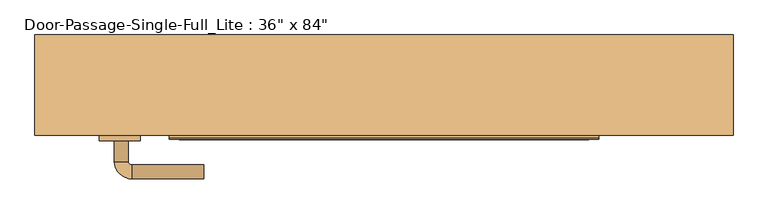
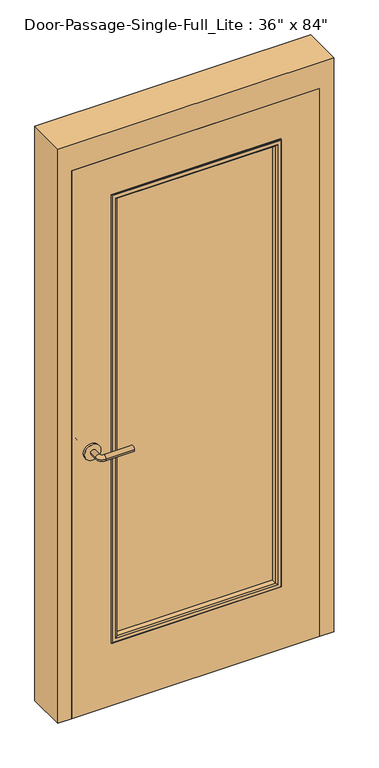
"""IFC4 building model written with IfcOpenShell, lengths in millimetres: door geometry."""

import ifcopenshell
import ifcopenshell.guid

model = None  # the IFC model being written
_history = None  # IfcOwnerHistory: only IFC2X3 demands one
_inside = {}  # id of a spatial element -> (the spatial element, [elements in it])
_under = {}  # id of a project, library or spatial element -> (it, [spatial elements below it])
_declared = {}  # id of a project -> (the project, [libraries it declares])
_typed = {}  # id of a type object -> (the type object, [elements of that type])
_made_of = {}  # id of a material, layer set ... -> (it, [elements and type objects made of it])


def new_model(schema):
    """Start an empty IFC model of exactly this schema.

    Asked for "IFC4X3", IfcOpenShell would pick the latest addendum, in which some entities
    have other attributes; the version numbers below select the first issue.
    IFC2X3 requires an IfcOwnerHistory on every rooted entity: one is made here for all.
    """
    global model, _history
    if schema == "IFC4X3":
        model = ifcopenshell.file(schema_version=(4, 3, 0, 0))
    else:
        model = ifcopenshell.file(schema=schema)
    _inside.clear()
    _under.clear()
    _declared.clear()
    _typed.clear()
    _made_of.clear()
    _history = None
    if model.schema == "IFC2X3":
        org = make("IfcOrganization", Name="unknown")
        user = make(
            "IfcPersonAndOrganization",
            ThePerson=make("IfcPerson", FamilyName="unknown"),
            TheOrganization=org,
        )
        app = make(
            "IfcApplication",
            ApplicationDeveloper=org,
            Version="unknown",
            ApplicationFullName="unknown",
            ApplicationIdentifier="unknown",
        )
        _history = make(
            "IfcOwnerHistory",
            OwningUser=user,
            OwningApplication=app,
            ChangeAction="ADDED",
            CreationDate=0,
        )
    return model


def make(cls, **values):
    """One entity of the class cls with the attributes given. An attribute that is None is left unset."""
    return model.create_entity(
        cls, **{name: value for name, value in values.items() if value is not None}
    )


def rooted(cls, **values):
    """An entity with a GlobalId (a new one), such as an element, a storey or a relation."""
    return make(cls, GlobalId=ifcopenshell.guid.new(), OwnerHistory=_history, **values)


def si_unit(unit_type, name, prefix=None):
    """IfcSIUnit, for example si_unit("LENGTHUNIT", "METRE", prefix="MILLI")."""
    return make("IfcSIUnit", UnitType=unit_type, Prefix=prefix, Name=name)


def assignment(units):
    """IfcUnitAssignment: the units of a project."""
    return None if units is None else make("IfcUnitAssignment", Units=units)


def point(xyz):
    """IfcCartesianPoint."""
    return None if xyz is None else make("IfcCartesianPoint", Coordinates=xyz)


def direction(xyz):
    """IfcDirection."""
    return None if xyz is None else make("IfcDirection", DirectionRatios=xyz)


def frame(location, z_axis=None, x_axis=None):
    """IfcAxis2Placement3D, a coordinate frame: its origin and axes. An axis left out is left unset."""
    return make(
        "IfcAxis2Placement3D",
        Location=point(location),
        Axis=direction(z_axis),
        RefDirection=direction(x_axis),
    )


def frame_2d(location, x_axis=None):
    """IfcAxis2Placement2D, a coordinate frame in the plane: its origin and x axis."""
    return make(
        "IfcAxis2Placement2D", Location=point(location), RefDirection=direction(x_axis)
    )


def origin():
    """The frame at (0, 0, 0) with its axes left unset."""
    return frame((0.0, 0.0, 0.0))


def place(relative_to, where):
    """IfcLocalPlacement: puts the frame where relative to a parent placement (None: the world)."""
    return make(
        "IfcLocalPlacement", PlacementRelTo=relative_to, RelativePlacement=where
    )


def context(
    kind, dimensions, precision=None, world=None, true_north=None, identifier=None
):
    """IfcGeometricRepresentationContext, for example the 3D "Model" context."""
    return make(
        "IfcGeometricRepresentationContext",
        ContextIdentifier=identifier,
        ContextType=kind,
        CoordinateSpaceDimension=dimensions,
        Precision=precision,
        WorldCoordinateSystem=world,
        TrueNorth=true_north,
    )


def project(units=None, contexts=None):
    """IfcProject with its units and contexts."""
    return rooted(
        "IfcProject",
        Name="project",
        RepresentationContexts=contexts,
        UnitsInContext=assignment(units),
    )


def spatial(cls, under=None, at=None, **own):
    """A site, building, storey or space (cls), placed at a placement, below another one or the project."""
    s = rooted(cls, ObjectPlacement=at, **own)
    if under is not None:
        _under.setdefault(under.id(), (under, []))[1].append(s)
    return s


def polyline(points):
    """IfcPolyline through the points."""
    return make("IfcPolyline", Points=[point(p) for p in points])


def circle_curve(where, radius):
    """IfcCircle in the frame where."""
    return make("IfcCircle", Position=where, Radius=radius)


def ellipse_curve(where, semi_axis1, semi_axis2):
    """IfcEllipse in the frame where."""
    return make(
        "IfcEllipse", Position=where, SemiAxis1=semi_axis1, SemiAxis2=semi_axis2
    )


def trimmed(basis, trim1, trim2, sense, master):
    """IfcTrimmedCurve: the piece of a basis curve between two trims."""
    return make(
        "IfcTrimmedCurve",
        BasisCurve=basis,
        Trim1=trim1,
        Trim2=trim2,
        SenseAgreement=sense,
        MasterRepresentation=master,
    )


def segment(curve, same_sense, transition):
    """IfcCompositeCurveSegment."""
    return make(
        "IfcCompositeCurveSegment",
        Transition=transition,
        SameSense=same_sense,
        ParentCurve=curve,
    )


def composite_curve(segments, self_intersect=None):
    """IfcCompositeCurve: segments joined end to end."""
    return make("IfcCompositeCurve", Segments=segments, SelfIntersect=self_intersect)


def outline(outer, holes=None, kind="AREA"):
    """IfcArbitraryClosedProfileDef: a profile drawn as a closed curve; with holes, ...WithVoids."""
    if holes is None:
        return make("IfcArbitraryClosedProfileDef", ProfileType=kind, OuterCurve=outer)
    return make(
        "IfcArbitraryProfileDefWithVoids",
        ProfileType=kind,
        OuterCurve=outer,
        InnerCurves=holes,
    )


def extrude(swept, where, along, depth):
    """IfcExtrudedAreaSolid: the profile swept, set in the frame where, extruded along a direction by depth."""
    return make(
        "IfcExtrudedAreaSolid",
        SweptArea=swept,
        Position=where,
        ExtrudedDirection=direction(along),
        Depth=depth,
    )


def faces_of(points, faces, orient=None, outer=None):
    """IfcFace entities. A face is a list of loops; a loop is a list of indices into points, from 0.

    orient and outer hold one flag for each loop. By default every Orientation is true, the
    first loop of a face is its IfcFaceOuterBound and the others are IfcFaceBound.
    """
    made = []
    for i, loops in enumerate(faces):
        bounds = []
        for j, loop in enumerate(loops):
            is_outer = j == 0 if outer is None else outer[i][j]
            bounds.append(
                make(
                    "IfcFaceOuterBound" if is_outer else "IfcFaceBound",
                    Bound=make("IfcPolyLoop", Polygon=[points[k] for k in loop]),
                    Orientation=True if orient is None else orient[i][j],
                )
            )
        made.append(make("IfcFace", Bounds=bounds))
    return made


def faceted_brep(points, faces, orient=None, outer=None, voids=None):
    """IfcFacetedBrep: a solid bounded by flat faces; with voids (closed shells), ...WithVoids."""
    shared = [point(p) for p in points]
    hull = make("IfcClosedShell", CfsFaces=faces_of(shared, faces, orient, outer))
    if voids is None:
        return make("IfcFacetedBrep", Outer=hull)
    return make(
        "IfcFacetedBrepWithVoids",
        Outer=hull,
        Voids=[
            make(cls, CfsFaces=faces_of(shared, fs, o, b)) for cls, fs, o, b in voids
        ],
    )


def shape(context_of_items, identifier, shape_type, items):
    """IfcShapeRepresentation: the items that make up one representation, for example the "Body"."""
    return make(
        "IfcShapeRepresentation",
        ContextOfItems=context_of_items,
        RepresentationIdentifier=identifier,
        RepresentationType=shape_type,
        Items=items,
    )


def source(mapping_origin, context_of_items, identifier, shape_type, items):
    """IfcRepresentationMap: a shape defined once, which mapped items show again and again."""
    return make(
        "IfcRepresentationMap",
        MappingOrigin=mapping_origin,
        MappedRepresentation=shape(context_of_items, identifier, shape_type, items),
    )


def transform(
    local_origin,
    x_axis=None,
    y_axis=None,
    z_axis=None,
    scale=None,
    scale2=None,
    scale3=None,
    uniform=True,
):
    """IfcCartesianTransformationOperator3D, or its non-uniform kind. x_axis, y_axis, z_axis: its Axis1, 2, 3."""
    if uniform:
        return make(
            "IfcCartesianTransformationOperator3D",
            Axis1=direction(x_axis),
            Axis2=direction(y_axis),
            LocalOrigin=point(local_origin),
            Scale=scale,
            Axis3=direction(z_axis),
        )
    return make(
        "IfcCartesianTransformationOperator3DnonUniform",
        Axis1=direction(x_axis),
        Axis2=direction(y_axis),
        LocalOrigin=point(local_origin),
        Scale=scale,
        Axis3=direction(z_axis),
        Scale2=scale2,
        Scale3=scale3,
    )


def mapped(mapping_source, mapping_target):
    """IfcMappedItem: shows the shape of a source again, moved by a transform."""
    return make(
        "IfcMappedItem", MappingSource=mapping_source, MappingTarget=mapping_target
    )


def made_of(thing, what):
    """Note that an element or type object is made of a material, layer set ...; save() writes the relation."""
    if what is not None:
        _made_of.setdefault(what.id(), (what, []))[1].append(thing)
    return thing


def element(
    cls,
    number,
    at=None,
    inside=None,
    cuts=None,
    type_object=None,
    material=None,
    context=None,
    identifier="Body",
    shape_type=None,
    held_by="IfcProductDefinitionShape",
    body=None,
    shapes=None,
    **own,
):
    """One element of the class cls, such as IfcWall. Its Tag is "e" and its number.

    at: its placement. inside: the storey or other place that contains it. cuts: it is an
    opening in that element (IfcRelVoidsElement). A single representation is given by context,
    identifier, shape_type and body (its items); several are given by shapes. held_by: the class
    of the entity that holds the representations. save() writes the other relations.
    """
    e = rooted(cls, Tag="e%d" % number, ObjectPlacement=at, **own)
    if body is not None:
        shapes = [shape(context, identifier, shape_type, body)]
    if shapes is not None:
        e.Representation = make(held_by, Representations=shapes)
    if inside is not None:
        _inside.setdefault(inside.id(), (inside, []))[1].append(e)
    if cuts is not None:
        rooted(
            "IfcRelVoidsElement", RelatingBuildingElement=cuts, RelatedOpeningElement=e
        )
    if type_object is not None:
        _typed.setdefault(type_object.id(), (type_object, []))[1].append(e)
    return made_of(e, material)


def aggregate(whole, parts):
    """IfcRelAggregates: a whole, such as a stair, and the parts it consists of."""
    return rooted("IfcRelAggregates", RelatingObject=whole, RelatedObjects=parts)


def save(model, path):
    """Write the relations noted so far, then the file.

    IfcRelAggregates (storeys below a building ...), IfcRelContainedInSpatialStructure (elements
    in a storey), IfcRelDefinesByType, IfcRelAssociatesMaterial and IfcRelDeclares: one each for
    every whole, place, type object, material and project.
    """
    for whole, parts in _under.values():
        aggregate(whole, parts)
    for where, things in _inside.values():
        rooted(
            "IfcRelContainedInSpatialStructure",
            RelatedElements=things,
            RelatingStructure=where,
        )
    for kind, things in _typed.values():
        rooted("IfcRelDefinesByType", RelatedObjects=things, RelatingType=kind)
    for what, things in _made_of.values():
        rooted("IfcRelAssociatesMaterial", RelatedObjects=things, RelatingMaterial=what)
    for by, libraries in _declared.values():
        rooted("IfcRelDeclares", RelatingContext=by, RelatedDefinitions=libraries)
    model.write(path)


def plane_surface(at):
    """IfcPlane: the flat surface through the origin of the frame at, square to its z axis."""
    return make("IfcPlane", Position=at)


def cylinder_surface(at, radius):
    """IfcCylindricalSurface: all points at the distance radius from the z axis of the frame at."""
    return make("IfcCylindricalSurface", Position=at, Radius=radius)


def revolved_surface(curve, axis_point, axis_direction):
    """IfcSurfaceOfRevolution: the curve turned about the line through axis_point along axis_direction."""
    return make(
        "IfcSurfaceOfRevolution",
        SweptCurve=make("IfcArbitraryOpenProfileDef", ProfileType="CURVE", Curve=curve),
        AxisPosition=make("IfcAxis1Placement", Location=point(axis_point), Axis=direction(axis_direction)),
    )


def advanced_brep(points, edges, surfaces, faces):
    """IfcAdvancedBrep: a solid bounded by faces that lie on surfaces and meet in shared edges.

    An edge is (start, end): straight between two places in points (the first is 0);
    or (start, end, curve); or (start, end, curve, False) where it runs against its curve.
    A face is (place in surfaces, loops), or (place, loops, False) where it looks against
    its surface's normal. A loop lists edges by number (the first is 1), with a minus sign
    where the edge is run from its end to its start. The first loop is the outer one.
    """
    corners = [point(p) for p in points]
    vertices = [make("IfcVertexPoint", VertexGeometry=c) for c in corners]
    made = []
    for start, end, *more in edges:
        made.append(
            make(
                "IfcEdgeCurve",
                EdgeStart=vertices[start],
                EdgeEnd=vertices[end],
                EdgeGeometry=more[0] if more else make("IfcPolyline", Points=[corners[start], corners[end]]),
                SameSense=more[1] if len(more) > 1 else True,
            )
        )
    hull = []
    for where, loops, *sense in faces:
        bounds = []
        for j, loop in enumerate(loops):
            ring = [make("IfcOrientedEdge", EdgeElement=made[abs(k) - 1], Orientation=k > 0) for k in loop]
            bounds.append(
                make(
                    "IfcFaceOuterBound" if j == 0 else "IfcFaceBound",
                    Bound=make("IfcEdgeLoop", EdgeList=ring),
                    Orientation=True,
                )
            )
        hull.append(make("IfcAdvancedFace", Bounds=bounds, FaceSurface=surfaces[where], SameSense=sense[0] if sense else True))
    return make("IfcAdvancedBrep", Outer=make("IfcClosedShell", CfsFaces=hull))


def door_58f93f42(model_context):
    return source(origin(), model_context, "Body", "SolidModel", [
        advanced_brep(
        [(-392.190625, 1.65, 1016.0), (-372.190625, 1.65, 1016.0), (-392.190625, 31.65, 1016.0), (-372.190625, 31.65, 1016.0), (-367.190625, 36.65, 1016.0), (-367.190625, 56.65, 1016.0), (-262.190625, 56.65, 1016.0), (-262.190625, 36.65, 1016.0)],
        [
            (0, 1, circle_curve(frame((-382.190625, 1.65, 1016.0), z_axis=(0.0, -1.0, 0.0), x_axis=(1.0, 0.0, 0.0)), 10.0)),
            (1, 0, circle_curve(frame((-382.190625, 1.65, 1016.0), z_axis=(0.0, -1.0, 0.0), x_axis=(1.0, 0.0, 0.0)), 10.0)),
            (0, 2),
            (2, 3, circle_curve(frame((-382.190625, 31.65, 1016.0), z_axis=(0.0, -1.0, 0.0), x_axis=(1.0, 0.0, 0.0)), 10.0)),
            (3, 1),
            (3, 2, circle_curve(frame((-382.190625, 31.65, 1016.0), z_axis=(0.0, -1.0, 0.0), x_axis=(1.0, 0.0, 0.0)), 10.0)),
            (4, 3, circle_curve(frame((-367.190625, 31.65, 1016.0), z_axis=(0.0, 0.0, 1.0), x_axis=(-1.0, 0.0, 0.0)), 5.0)),
            (2, 5, circle_curve(frame((-367.190625, 31.65, 1016.0), z_axis=(0.0, 0.0, -1.0), x_axis=(-1.0, 0.0, 0.0)), 25.0)),
            (5, 4, circle_curve(frame((-367.190625, 46.65, 1016.0), z_axis=(-1.0, 0.0, 0.0), x_axis=(0.0, -1.0, 0.0)), 10.0)),
            (4, 5, circle_curve(frame((-367.190625, 46.65, 1016.0), z_axis=(-1.0, 0.0, 0.0), x_axis=(0.0, -1.0, 0.0)), 10.0)),
            (6, 7, circle_curve(frame((-262.190625, 46.65, 1016.0), z_axis=(1.0, 0.0, 0.0), x_axis=(0.0, -1.0, 0.0)), 10.0)),
            (7, 6, circle_curve(frame((-262.190625, 46.65, 1016.0), z_axis=(1.0, 0.0, 0.0), x_axis=(0.0, -1.0, 0.0)), 10.0)),
            (5, 6),
            (7, 4),
        ],
        [
            plane_surface(frame((-382.190625, 1.65, 1016.0), z_axis=(0.0, -1.0, 0.0), x_axis=(0.0, 0.0, 1.0))),
            cylinder_surface(frame((-382.190625, 1.65, 1016.0), z_axis=(0.0, -1.0, 0.0), x_axis=(1.0, 0.0, 0.0)), 10.0),
            revolved_surface(trimmed(ellipse_curve(frame((-382.190625, 31.65, 1016.0), z_axis=(0.0, -1.0, 0.0), x_axis=(1.0, 0.0, 0.0)), 10.0, 10.0), [point((-392.190625, 31.65, 1016.0))], [point((-372.190625, 31.65, 1016.0))], True, "CARTESIAN"), (-367.190625, 31.65, 1016.0), (0.0, 0.0, -1.0)),
            revolved_surface(trimmed(ellipse_curve(frame((-382.190625, 31.65, 1016.0), z_axis=(0.0, -1.0, 0.0), x_axis=(1.0, 0.0, 0.0)), 10.0, 10.0), [point((-372.190625, 31.65, 1016.0))], [point((-392.190625, 31.65, 1016.0))], True, "CARTESIAN"), (-367.190625, 31.65, 1016.0), (0.0, 0.0, -1.0)),
            plane_surface(frame((-262.190625, 46.65, 1016.0), z_axis=(1.0, 0.0, 0.0), x_axis=(0.0, 0.0, 1.0))),
            cylinder_surface(frame((-367.190625, 46.65, 1016.0), z_axis=(-1.0, 0.0, 0.0), x_axis=(0.0, -1.0, 0.0)), 10.0),
        ],
        [
            (0, [[1, 2]]),
            (1, [[-1, 3, 4, 5]]),
            (1, [[-2, -5, 6, -3]]),
            (2, [[7, -4, 8, 9]]),
            (3, [[-8, -6, -7, 10]]),
            (4, [[11, 12]]),
            (5, [[-9, 13, -12, 14]]),
            (5, [[-10, -14, -11, -13]]),
        ],
    ),
        extrude(outline(composite_curve([segment(trimmed(circle_curve(frame_2d((1016.0, -384.690625)), 30.0), [point((1016.0, -414.690625))], [point((1016.0, -354.690625))], False, "CARTESIAN"), True, "CONTINUOUS"), segment(trimmed(circle_curve(frame_2d((1016.0, -384.690625)), 30.0), [point((1016.0, -354.690625))], [point((1016.0, -414.690625))], False, "CARTESIAN"), True, "CONTINUOUS")], self_intersect=False)), frame((0.0, -6.35, 0.0), z_axis=(0.0, 1.0, 0.0), x_axis=(0.0, 0.0, 1.0)), (0.0, 0.0, 1.0), 8.0),
        advanced_brep(
        [(-392.190625, -58.8, 1016.0), (-372.190625, -58.8, 1016.0), (-372.190625, -88.8, 1016.0), (-392.190625, -88.8, 1016.0), (-367.190625, -93.8, 1016.0), (-367.190625, -113.8, 1016.0), (-262.190625, -113.8, 1016.0), (-262.190625, -93.8, 1016.0)],
        [
            (0, 1, circle_curve(frame((-382.190625, -58.8, 1016.0), z_axis=(0.0, 1.0, 0.0), x_axis=(1.0, 0.0, 0.0)), 10.0)),
            (1, 0, circle_curve(frame((-382.190625, -58.8, 1016.0), z_axis=(0.0, 1.0, 0.0), x_axis=(1.0, 0.0, 0.0)), 10.0)),
            (1, 2),
            (2, 3, circle_curve(frame((-382.190625, -88.8, 1016.0), z_axis=(0.0, 1.0, 0.0), x_axis=(1.0, 0.0, 0.0)), 10.0)),
            (3, 0),
            (3, 2, circle_curve(frame((-382.190625, -88.8, 1016.0), z_axis=(0.0, 1.0, 0.0), x_axis=(1.0, 0.0, 0.0)), 10.0)),
            (4, 5, circle_curve(frame((-367.190625, -103.8, 1016.0), z_axis=(-1.0, 0.0, 0.0), x_axis=(0.0, 1.0, 0.0)), 10.0)),
            (5, 3, circle_curve(frame((-367.190625, -88.8, 1016.0), z_axis=(0.0, 0.0, -1.0), x_axis=(-1.0, 0.0, 0.0)), 25.0)),
            (2, 4, circle_curve(frame((-367.190625, -88.8, 1016.0), z_axis=(0.0, 0.0, 1.0), x_axis=(-1.0, 0.0, 0.0)), 5.0)),
            (5, 4, circle_curve(frame((-367.190625, -103.8, 1016.0), z_axis=(-1.0, 0.0, 0.0), x_axis=(0.0, 1.0, 0.0)), 10.0)),
            (6, 7, circle_curve(frame((-262.190625, -103.8, 1016.0), z_axis=(1.0, 0.0, 0.0), x_axis=(0.0, 1.0, 0.0)), 10.0)),
            (7, 6, circle_curve(frame((-262.190625, -103.8, 1016.0), z_axis=(1.0, 0.0, 0.0), x_axis=(0.0, 1.0, 0.0)), 10.0)),
            (4, 7),
            (6, 5),
        ],
        [
            plane_surface(frame((-382.190625, -58.8, 1016.0), z_axis=(0.0, 1.0, 0.0), x_axis=(0.0, 0.0, 1.0))),
            cylinder_surface(frame((-382.190625, -58.8, 1016.0), z_axis=(0.0, 1.0, 0.0), x_axis=(1.0, 0.0, 0.0)), 10.0),
            revolved_surface(trimmed(ellipse_curve(frame((-382.190625, -88.8, 1016.0), z_axis=(0.0, -1.0, 0.0), x_axis=(1.0, 0.0, 0.0)), 10.0, 10.0), [point((-392.190625, -88.8, 1016.0))], [point((-372.190625, -88.8, 1016.0))], True, "CARTESIAN"), (-367.190625, -88.8, 1016.0), (0.0, 0.0, -1.0)),
            revolved_surface(trimmed(ellipse_curve(frame((-382.190625, -88.8, 1016.0), z_axis=(0.0, -1.0, 0.0), x_axis=(1.0, 0.0, 0.0)), 10.0, 10.0), [point((-372.190625, -88.8, 1016.0))], [point((-392.190625, -88.8, 1016.0))], True, "CARTESIAN"), (-367.190625, -88.8, 1016.0), (0.0, 0.0, -1.0)),
            plane_surface(frame((-262.190625, -103.8, 1016.0), z_axis=(1.0, 0.0, 0.0), x_axis=(0.0, 0.0, 1.0))),
            cylinder_surface(frame((-367.190625, -103.8, 1016.0), z_axis=(-1.0, 0.0, 0.0), x_axis=(0.0, 1.0, 0.0)), 10.0),
        ],
        [
            (0, [[1, 2]]),
            (1, [[3, 4, 5, -2]]),
            (1, [[-5, 6, -3, -1]]),
            (2, [[7, 8, -4, 9]]),
            (3, [[10, -9, -6, -8]]),
            (4, [[11, 12]]),
            (5, [[13, -11, 14, -7]]),
            (5, [[-14, -12, -13, -10]]),
        ],
    ),
        extrude(outline(composite_curve([segment(trimmed(circle_curve(frame_2d((1016.0, -384.690625)), 30.0), [point((1016.0, -414.690625))], [point((1016.0, -354.690625))], False, "CARTESIAN"), True, "CONTINUOUS"), segment(trimmed(circle_curve(frame_2d((1016.0, -384.690625)), 30.0), [point((1016.0, -354.690625))], [point((1016.0, -414.690625))], False, "CARTESIAN"), True, "CONTINUOUS")], self_intersect=False)), frame((0.0, -58.8, 0.0), z_axis=(0.0, 1.0, 0.0), x_axis=(0.0, 0.0, 1.0)), (0.0, 0.0, 1.0), 8.0),
        extrude(outline(polyline([(304.8, -25.4), (304.8, -31.75), (-304.8, -31.75), (-304.8, -25.4), (304.8, -25.4)])), frame((0.0, 0.0, 254.0), z_axis=(0.0, 0.0, 1.0), x_axis=(1.0, 0.0, 0.0)), (0.0, 0.0, 1.0), 1727.2),
        faceted_brep([(457.2, -1.5875, 0.0), (441.325, -1.5875, 0.0), (441.325, 46.0375, 0.0), (457.2, 46.0375, 0.0), (457.2, 95.25, 0.0), (508.0, 95.25, 0.0), (508.0, -50.8, 0.0), (457.2, -50.8, 0.0), (457.2, -50.8, 2133.6), (457.2, -1.5875, 2133.6), (508.0, -50.8, 2235.2), (-508.0, -50.8, 2235.2), (-508.0, -50.8, 0.0), (-457.2, -50.8, 0.0), (-457.2, -50.8, 2133.6), (508.0, 95.25, 2235.2), (457.2, 95.25, 2133.6), (-457.2, 95.25, 2133.6), (-457.2, 95.25, 0.0), (-508.0, 95.25, 0.0), (-508.0, 95.25, 2235.2), (457.2, 46.0375, 2133.6), (441.325, 46.0375, 2117.725), (-441.325, 46.0375, 2117.725), (-441.325, 46.0375, 0.0), (-457.2, 46.0375, 0.0), (-457.2, 46.0375, 2133.6), (441.325, -1.5875, 2117.725), (-457.2, -1.5875, 2133.6), (-457.2, -1.5875, 0.0), (-441.325, -1.5875, 0.0), (-441.325, -1.5875, 2117.725)], [[[0, 1, 2, 3, 4, 5, 6, 7]], [[7, 8, 9, 0]], [[6, 10, 11, 12, 13, 14, 8, 7]], [[5, 15, 10, 6]], [[4, 16, 17, 18, 19, 20, 15, 5]], [[3, 21, 16, 4]], [[2, 22, 23, 24, 25, 26, 21, 3]], [[1, 27, 22, 2]], [[0, 9, 28, 29, 30, 31, 27, 1]], [[8, 14, 28, 9]], [[16, 21, 26, 17]], [[22, 27, 31, 23]], [[12, 19, 18, 25, 24, 30, 29, 13]], [[13, 29, 28, 14]], [[11, 20, 19, 12]], [[17, 26, 25, 18]], [[23, 31, 30, 24]], [[15, 20, 11, 10]]]),
        extrude(outline(polyline([(2133.6, -457.2), (0.0, -457.2), (0.0, 457.2), (2133.6, 457.2), (2133.6, -457.2)]), holes=[polyline([(1981.2, -304.8), (1981.2, 304.8), (254.0, 304.8), (254.0, -304.8), (1981.2, -304.8)])]), frame((0.0, -50.8, 0.0), z_axis=(0.0, 1.0, 0.0), x_axis=(0.0, 0.0, 1.0)), (0.0, 0.0, 1.0), 44.45),
        advanced_brep(
        [(-304.8, -31.75, 1981.2), (-304.8, -31.75, 254.0), (-304.8, -50.8, 254.0), (-304.8, -50.8, 1981.2), (-292.8, -51.8, 1969.2), (-292.8, -51.8, 266.0), (-292.8, -31.75, 266.0), (-292.8, -31.75, 1969.2), (-297.8, -56.8, 1974.2), (-297.8, -56.8, 261.0), (-312.8, -54.8, 1989.2), (-312.8, -54.8, 246.0), (-310.8, -56.8, 248.0), (-310.8, -56.8, 1987.2), (-312.8, -50.8, 1989.2), (-312.8, -50.8, 246.0), (304.8, -31.75, 254.0), (304.8, -50.8, 254.0), (292.8, -51.8, 266.0), (292.8, -31.75, 266.0), (297.8, -56.8, 261.0), (312.8, -54.8, 246.0), (310.8, -56.8, 248.0), (312.8, -50.8, 246.0), (304.8, -31.75, 1981.2), (304.8, -50.8, 1981.2), (292.8, -51.8, 1969.2), (292.8, -31.75, 1969.2), (297.8, -56.8, 1974.2), (312.8, -54.8, 1989.2), (310.8, -56.8, 1987.2), (312.8, -50.8, 1989.2)],
        [
            (0, 1),
            (1, 2),
            (2, 3),
            (3, 0),
            (4, 5),
            (5, 6),
            (6, 7),
            (7, 4),
            (8, 9),
            (9, 5, ellipse_curve(frame((-297.8, -51.8, 261.0), z_axis=(-0.7071067811865475, 0.0, 0.7071067811865475), x_axis=(0.7071067811865474, 0.0, 0.7071067811865476)), 7.0710678, 5.0)),
            (4, 8, ellipse_curve(frame((-297.8, -51.8, 1974.2), z_axis=(-0.7071067811865475, 0.0, -0.7071067811865475), x_axis=(-0.7071067811865474, 0.0, 0.7071067811865476)), 7.0710678, 5.0)),
            (10, 11),
            (11, 12, ellipse_curve(frame((-310.8, -54.8, 248.0), z_axis=(-0.7071067811865475, 0.0, 0.7071067811865475), x_axis=(0.7071067811865474, 0.0, 0.7071067811865476)), 2.8284271, 2.0)),
            (12, 13),
            (13, 10, ellipse_curve(frame((-310.8, -54.8, 1987.2), z_axis=(-0.7071067811865475, 0.0, -0.7071067811865475), x_axis=(-0.7071067811865474, 0.0, 0.7071067811865476)), 2.8284271, 2.0)),
            (14, 15),
            (15, 11),
            (10, 14),
            (1, 16),
            (16, 17),
            (17, 2),
            (5, 18),
            (18, 19),
            (19, 6),
            (9, 20),
            (20, 18, ellipse_curve(frame((297.8, -51.8, 261.0), z_axis=(-0.7071067811865475, 0.0, -0.7071067811865475), x_axis=(-0.7071067811865476, 0.0, 0.7071067811865474)), 7.0710678, 5.0)),
            (11, 21),
            (21, 22, ellipse_curve(frame((310.8, -54.8, 248.0), z_axis=(-0.7071067811865475, 0.0, -0.7071067811865475), x_axis=(-0.7071067811865476, 0.0, 0.7071067811865474)), 2.8284271, 2.0)),
            (22, 12),
            (15, 23),
            (23, 21),
            (16, 24),
            (24, 25),
            (25, 17),
            (18, 26),
            (26, 27),
            (27, 19),
            (20, 28),
            (28, 26, ellipse_curve(frame((297.8, -51.8, 1974.2), z_axis=(0.7071067811865475, 0.0, -0.7071067811865475), x_axis=(-0.7071067811865474, 0.0, -0.7071067811865476)), 7.0710678, 5.0)),
            (21, 29),
            (29, 30, ellipse_curve(frame((310.8, -54.8, 1987.2), z_axis=(0.7071067811865475, 0.0, -0.7071067811865475), x_axis=(-0.7071067811865474, 0.0, -0.7071067811865476)), 2.8284271, 2.0)),
            (30, 22),
            (23, 31),
            (31, 29),
            (14, 31),
            (25, 3),
            (24, 0),
            (27, 7),
            (26, 4),
            (28, 8),
            (30, 13),
            (29, 10),
        ],
        [
            plane_surface(frame((-304.8, -50.8, 1981.2), z_axis=(-1.0, 0.0, 0.0), x_axis=(0.0, 0.0, -1.0))),
            plane_surface(frame((-292.8, -31.75, 1969.2), z_axis=(1.0, 0.0, 0.0), x_axis=(0.0, 0.0, -1.0))),
            cylinder_surface(frame((-297.8, -51.8, 1981.2), z_axis=(0.0, 0.0, 1.0), x_axis=(-1.0, 0.0, 0.0)), 5.0),
            cylinder_surface(frame((-310.8, -54.8, 1981.2), z_axis=(0.0, 0.0, 1.0), x_axis=(-1.0, 0.0, 0.0)), 2.0),
            plane_surface(frame((-312.8, -54.8, 1989.2), z_axis=(-1.0, 0.0, 0.0), x_axis=(0.0, 0.0, -1.0))),
            plane_surface(frame((-304.8, -50.8, 254.0), z_axis=(0.0, 0.0, -1.0), x_axis=(1.0, 0.0, 0.0))),
            plane_surface(frame((-292.8, -31.75, 266.0), z_axis=(0.0, 0.0, 1.0), x_axis=(1.0, 0.0, 0.0))),
            cylinder_surface(frame((-304.8, -51.8, 261.0), z_axis=(-1.0, 0.0, 0.0), x_axis=(0.0, 0.0, -1.0)), 5.0),
            cylinder_surface(frame((-304.8, -54.8, 248.0), z_axis=(-1.0, 0.0, 0.0), x_axis=(0.0, 0.0, -1.0)), 2.0),
            plane_surface(frame((-312.8, -54.8, 246.0), z_axis=(0.0, 0.0, -1.0), x_axis=(1.0, 0.0, 0.0))),
            plane_surface(frame((304.8, -50.8, 254.0), z_axis=(1.0, 0.0, 0.0), x_axis=(0.0, 0.0, 1.0))),
            plane_surface(frame((292.8, -31.75, 266.0), z_axis=(-1.0, 0.0, 0.0), x_axis=(0.0, 0.0, 1.0))),
            cylinder_surface(frame((297.8, -51.8, 254.0), z_axis=(0.0, 0.0, -1.0), x_axis=(1.0, 0.0, 0.0)), 5.0),
            cylinder_surface(frame((310.8, -54.8, 254.0), z_axis=(0.0, 0.0, -1.0), x_axis=(1.0, 0.0, 0.0)), 2.0),
            plane_surface(frame((312.8, -54.8, 246.0), z_axis=(1.0, 0.0, 0.0), x_axis=(0.0, 0.0, 1.0))),
            plane_surface(frame((312.8, -50.8, 1989.2), z_axis=(0.0, 1.0, 0.0), x_axis=(-1.0, 0.0, 0.0))),
            plane_surface(frame((304.8, -50.8, 1981.2), z_axis=(0.0, 0.0, 1.0), x_axis=(-1.0, 0.0, 0.0))),
            plane_surface(frame((304.8, -31.75, 1981.2), z_axis=(0.0, 1.0, 0.0), x_axis=(-1.0, 0.0, 0.0))),
            plane_surface(frame((292.8, -31.75, 1969.2), z_axis=(0.0, 0.0, -1.0), x_axis=(-1.0, 0.0, 0.0))),
            cylinder_surface(frame((304.8, -51.8, 1974.2), z_axis=(1.0, 0.0, 0.0), x_axis=(0.0, 0.0, 1.0)), 5.0),
            plane_surface(frame((297.8, -56.8, 1974.2), z_axis=(0.0, -1.0, 0.0), x_axis=(-1.0, 0.0, 0.0))),
            cylinder_surface(frame((304.8, -54.8, 1987.2), z_axis=(1.0, 0.0, 0.0), x_axis=(0.0, 0.0, 1.0)), 2.0),
            plane_surface(frame((312.8, -54.8, 1989.2), z_axis=(0.0, 0.0, 1.0), x_axis=(-1.0, 0.0, 0.0))),
        ],
        [
            (0, [[1, 2, 3, 4]]),
            (1, [[5, 6, 7, 8]]),
            (2, [[9, 10, -5, 11]]),
            (3, [[12, 13, 14, 15]]),
            (4, [[16, 17, -12, 18]]),
            (5, [[19, 20, 21, -2]]),
            (6, [[22, 23, 24, -6]]),
            (7, [[25, 26, -22, -10]]),
            (8, [[27, 28, 29, -13]]),
            (9, [[30, 31, -27, -17]]),
            (10, [[32, 33, 34, -20]]),
            (11, [[35, 36, 37, -23]]),
            (12, [[38, 39, -35, -26]]),
            (13, [[40, 41, 42, -28]]),
            (14, [[43, 44, -40, -31]]),
            (15, [[-16, 45, -43, -30], [-3, -21, -34, 46]]),
            (16, [[47, -4, -46, -33]]),
            (17, [[-1, -47, -32, -19], [-7, -24, -37, 48]]),
            (18, [[49, -8, -48, -36]]),
            (19, [[50, -11, -49, -39]]),
            (20, [[-14, -29, -42, 51], [-9, -50, -38, -25]]),
            (21, [[52, -15, -51, -41]]),
            (22, [[-45, -18, -52, -44]]),
        ],
    ),
        advanced_brep(
        [(-304.8, -25.4, 254.0), (-304.8, -25.4, 1981.2), (-304.8, -6.35, 1981.2), (-304.8, -6.35, 254.0), (-292.8, -5.35, 266.0), (-292.8, -5.35, 1969.2), (-292.8, -25.4, 1969.2), (-292.8, -25.4, 266.0), (-297.8, -0.35, 261.0), (-297.8, -0.35, 1974.2), (-312.8, -2.35, 246.0), (-312.8, -2.35, 1989.2), (-310.8, -0.35, 1987.2), (-310.8, -0.35, 248.0), (-312.8, -6.35, 246.0), (-312.8, -6.35, 1989.2), (304.8, -25.4, 1981.2), (304.8, -6.35, 1981.2), (292.8, -5.35, 1969.2), (292.8, -25.4, 1969.2), (297.8, -0.35, 1974.2), (312.8, -2.35, 1989.2), (310.8, -0.35, 1987.2), (312.8, -6.35, 1989.2), (304.8, -25.4, 254.0), (304.8, -6.35, 254.0), (292.8, -5.35, 266.0), (292.8, -25.4, 266.0), (297.8, -0.35, 261.0), (312.8, -2.35, 246.0), (310.8, -0.35, 248.0), (312.8, -6.35, 246.0)],
        [
            (0, 1),
            (1, 2),
            (2, 3),
            (3, 0),
            (4, 5),
            (5, 6),
            (6, 7),
            (7, 4),
            (8, 9),
            (9, 5, ellipse_curve(frame((-297.8, -5.35, 1974.2), z_axis=(-0.7071067811865475, 0.0, -0.7071067811865475), x_axis=(0.7071067811865474, 0.0, -0.7071067811865476)), 7.0710678, 5.0)),
            (4, 8, ellipse_curve(frame((-297.8, -5.35, 261.0), z_axis=(-0.7071067811865475, 0.0, 0.7071067811865475), x_axis=(-0.7071067811865474, 0.0, -0.7071067811865476)), 7.0710678, 5.0)),
            (10, 11),
            (11, 12, ellipse_curve(frame((-310.8, -2.35, 1987.2), z_axis=(-0.7071067811865475, 0.0, -0.7071067811865475), x_axis=(0.7071067811865474, 0.0, -0.7071067811865476)), 2.8284271, 2.0)),
            (12, 13),
            (13, 10, ellipse_curve(frame((-310.8, -2.35, 248.0), z_axis=(-0.7071067811865475, 0.0, 0.7071067811865475), x_axis=(-0.7071067811865474, 0.0, -0.7071067811865476)), 2.8284271, 2.0)),
            (14, 15),
            (15, 11),
            (10, 14),
            (1, 16),
            (16, 17),
            (17, 2),
            (5, 18),
            (18, 19),
            (19, 6),
            (9, 20),
            (20, 18, ellipse_curve(frame((297.8, -5.35, 1974.2), z_axis=(-0.7071067811865475, 0.0, 0.7071067811865475), x_axis=(-0.7071067811865476, 0.0, -0.7071067811865474)), 7.0710678, 5.0)),
            (11, 21),
            (21, 22, ellipse_curve(frame((310.8, -2.35, 1987.2), z_axis=(-0.7071067811865475, 0.0, 0.7071067811865475), x_axis=(-0.7071067811865476, 0.0, -0.7071067811865474)), 2.8284271, 2.0)),
            (22, 12),
            (15, 23),
            (23, 21),
            (16, 24),
            (24, 25),
            (25, 17),
            (18, 26),
            (26, 27),
            (27, 19),
            (20, 28),
            (28, 26, ellipse_curve(frame((297.8, -5.35, 261.0), z_axis=(0.7071067811865475, 0.0, 0.7071067811865475), x_axis=(-0.7071067811865474, 0.0, 0.7071067811865476)), 7.0710678, 5.0)),
            (21, 29),
            (29, 30, ellipse_curve(frame((310.8, -2.35, 248.0), z_axis=(0.7071067811865475, 0.0, 0.7071067811865475), x_axis=(-0.7071067811865474, 0.0, 0.7071067811865476)), 2.8284271, 2.0)),
            (30, 22),
            (23, 31),
            (31, 29),
            (14, 31),
            (25, 3),
            (24, 0),
            (27, 7),
            (26, 4),
            (28, 8),
            (30, 13),
            (29, 10),
        ],
        [
            plane_surface(frame((-304.8, -6.35, 254.0), z_axis=(-1.0, 0.0, 0.0), x_axis=(0.0, 0.0, 1.0))),
            plane_surface(frame((-292.8, -25.4, 266.0), z_axis=(1.0, 0.0, 0.0), x_axis=(0.0, 0.0, 1.0))),
            cylinder_surface(frame((-297.8, -5.35, 254.0), z_axis=(0.0, 0.0, -1.0), x_axis=(-1.0, 0.0, 0.0)), 5.0),
            cylinder_surface(frame((-310.8, -2.35, 254.0), z_axis=(0.0, 0.0, -1.0), x_axis=(-1.0, 0.0, 0.0)), 2.0),
            plane_surface(frame((-312.8, -2.35, 246.0), z_axis=(-1.0, 0.0, 0.0), x_axis=(0.0, 0.0, 1.0))),
            plane_surface(frame((-304.8, -6.35, 1981.2), z_axis=(0.0, 0.0, 1.0), x_axis=(1.0, 0.0, 0.0))),
            plane_surface(frame((-292.8, -25.4, 1969.2), z_axis=(0.0, 0.0, -1.0), x_axis=(1.0, 0.0, 0.0))),
            cylinder_surface(frame((-304.8, -5.35, 1974.2), z_axis=(-1.0, 0.0, 0.0), x_axis=(0.0, 0.0, 1.0)), 5.0),
            cylinder_surface(frame((-304.8, -2.35, 1987.2), z_axis=(-1.0, 0.0, 0.0), x_axis=(0.0, 0.0, 1.0)), 2.0),
            plane_surface(frame((-312.8, -2.35, 1989.2), z_axis=(0.0, 0.0, 1.0), x_axis=(1.0, 0.0, 0.0))),
            plane_surface(frame((304.8, -6.35, 1981.2), z_axis=(1.0, 0.0, 0.0), x_axis=(0.0, 0.0, -1.0))),
            plane_surface(frame((292.8, -25.4, 1969.2), z_axis=(-1.0, 0.0, 0.0), x_axis=(0.0, 0.0, -1.0))),
            cylinder_surface(frame((297.8, -5.35, 1981.2), z_axis=(0.0, 0.0, 1.0), x_axis=(1.0, 0.0, 0.0)), 5.0),
            cylinder_surface(frame((310.8, -2.35, 1981.2), z_axis=(0.0, 0.0, 1.0), x_axis=(1.0, 0.0, 0.0)), 2.0),
            plane_surface(frame((312.8, -2.35, 1989.2), z_axis=(1.0, 0.0, 0.0), x_axis=(0.0, 0.0, -1.0))),
            plane_surface(frame((312.8, -6.35, 246.0), z_axis=(0.0, -1.0, 0.0), x_axis=(-1.0, 0.0, 0.0))),
            plane_surface(frame((304.8, -6.35, 254.0), z_axis=(0.0, 0.0, -1.0), x_axis=(-1.0, 0.0, 0.0))),
            plane_surface(frame((304.8, -25.4, 254.0), z_axis=(0.0, -1.0, 0.0), x_axis=(-1.0, 0.0, 0.0))),
            plane_surface(frame((292.8, -25.4, 266.0), z_axis=(0.0, 0.0, 1.0), x_axis=(-1.0, 0.0, 0.0))),
            cylinder_surface(frame((304.8, -5.35, 261.0), z_axis=(1.0, 0.0, 0.0), x_axis=(0.0, 0.0, -1.0)), 5.0),
            plane_surface(frame((297.8, -0.35, 261.0), z_axis=(0.0, 1.0, 0.0), x_axis=(-1.0, 0.0, 0.0))),
            cylinder_surface(frame((304.8, -2.35, 248.0), z_axis=(1.0, 0.0, 0.0), x_axis=(0.0, 0.0, -1.0)), 2.0),
            plane_surface(frame((312.8, -2.35, 246.0), z_axis=(0.0, 0.0, -1.0), x_axis=(-1.0, 0.0, 0.0))),
        ],
        [
            (0, [[1, 2, 3, 4]]),
            (1, [[5, 6, 7, 8]]),
            (2, [[9, 10, -5, 11]]),
            (3, [[12, 13, 14, 15]]),
            (4, [[16, 17, -12, 18]]),
            (5, [[19, 20, 21, -2]]),
            (6, [[22, 23, 24, -6]]),
            (7, [[25, 26, -22, -10]]),
            (8, [[27, 28, 29, -13]]),
            (9, [[30, 31, -27, -17]]),
            (10, [[32, 33, 34, -20]]),
            (11, [[35, 36, 37, -23]]),
            (12, [[38, 39, -35, -26]]),
            (13, [[40, 41, 42, -28]]),
            (14, [[43, 44, -40, -31]]),
            (15, [[-16, 45, -43, -30], [-3, -21, -34, 46]]),
            (16, [[47, -4, -46, -33]]),
            (17, [[-1, -47, -32, -19], [-7, -24, -37, 48]]),
            (18, [[49, -8, -48, -36]]),
            (19, [[50, -11, -49, -39]]),
            (20, [[-14, -29, -42, 51], [-9, -50, -38, -25]]),
            (21, [[52, -15, -51, -41]]),
            (22, [[-45, -18, -52, -44]]),
        ],
    ),
    ])


if __name__ == "__main__":
    model = new_model("IFC4")
    model_context = context("Model", 3, world=origin())
    ifc_project = project(units=[si_unit("LENGTHUNIT", "METRE", prefix="MILLI")], contexts=[model_context])
    site = spatial("IfcSite", under=ifc_project)
    building = spatial("IfcBuilding", under=site)
    placement = place(None, origin())
    door_shape = door_58f93f42(model_context)
    element("IfcDoor", 1, ObjectType="Door-Passage-Single-Full_Lite : 36\" x 84\"", at=placement, inside=building, context=model_context, shape_type="MappedRepresentation", body=[
        mapped(door_shape, transform((0.0, 0.0, 0.0), x_axis=(1.0, 0.0, 0.0), y_axis=(0.0, 1.0, 0.0), z_axis=(0.0, 0.0, 1.0))),
    ])
    save(model, "model.ifc")

# Revit data of these elements
# Type "Door-Passage-Single-Full_Lite : 36\" x 84\""
#   Type Mark = "52"
#   Assembly Code = "B2030100"
#   Analytic Construction = "Wooden"
#   Thickness = 0' - 1 3/4"
#   Thermal Resistance (R) = 2.5876 (h·ft²·°F)/BTU
#   Swing Angle [instance default] = 90.00°
#   Strike Height = 3' - 4"
#   Rough Width [instance default] = 3' - 4"
#   Rough Height [instance default] = 7' - 4"
#   MF Opening Height [instance default] = 0' - 4"
#   MF Opening Width [instance default] = 0' - 4"
#   Inset Calculate [instance default] = 0' - 4"
#   Masonry Inset [instance default] = 0' - 1"
#   Height = 7' - 0"
#   Width = 3' - 0"
#   Heat Transfer Coefficient (U) = 0.3865 BTU/(h·ft²·°F)
#   Masonry Frame Depth = 0' - 5 3/4"
#   Masonry Frame [instance default] = yes
#   Function = 1
#   Dry Wall Frame [instance default] = no
#   Panel Material = Wood - Birch
#   Glazing = Glass
#   Glass Stop Material = Metal - Paint Finish - Grey
#   Frame Material = Metal - Paint Finish - Grey
#   Door Handle Material = Aluminum
#   Visual Light Transmittance = 0
#   Solar Heat Gain Coefficient = 0
#   Wall Closure = (empty or 0)
# Element 1 (IfcDoor, "Door-Passage-Single-Full_Lite : 36\" x 84\"")
#   Materials on its faces: "Metal - Paint Finish - Grey", "Aluminum", "Wood - Birch", "Glass"
# Materials
#   "Wood - Birch": class "Wood", colour RGB 166 116 52, transparency 0, Cost = 0
#   "Glass": class "Glass", colour RGB 0 128 192, transparency 0.75, Description = "Soda Lime Glass", Cost = 0
#   "Metal - Paint Finish - Grey": class "Paint", colour RGB 104 104 104, transparency 0, Cost = 0
#   "Aluminum": class "Metal", colour RGB 247 247 247, transparency 0, Description = "Aluminum 6061", Cost = 0
